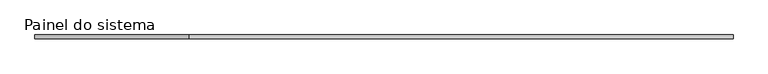
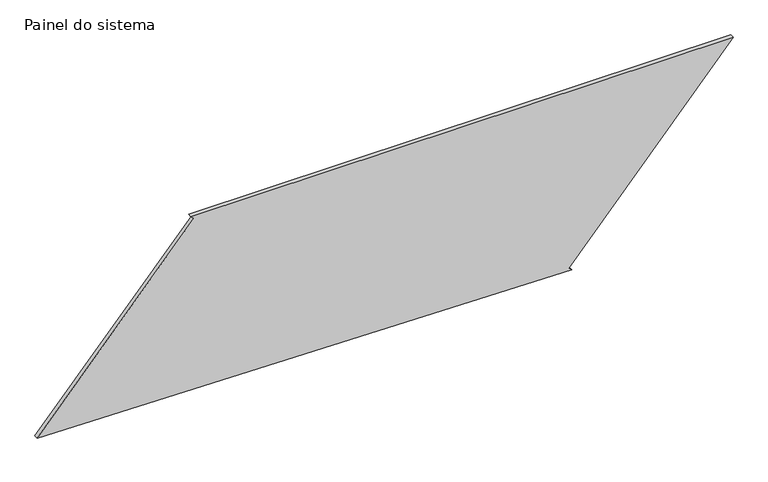
"""IFC4 building model written with IfcOpenShell, lengths in millimetres: plate geometry, Painel do sistema : Envidraçado."""

from ifc_helpers import new_model, si_unit, frame, origin, place, context, project, spatial, polyline, outline, extrude, source, transform, mapped, element, save


def painel_do_sistema_3713dc80(model_context):
    return source(origin(), model_context, "Body", "SweptSolid", [
        extrude(outline(polyline([(0.0, 1167.9821975), (16.5356636, 1149.2319488), (1185.4896941, 2180.1212412), (1185.4896941, -1216.67228), (1168.9540304, -1197.9220313), (55.2110382, -2180.1212412), (0.0, 1167.9821975)])), frame((0.0, 24.5, 0.0), z_axis=(0.0, 1.0, 0.0), x_axis=(0.0, 0.0, 1.0)), (0.0, 0.0, 1.0), 25.0),
    ])


if __name__ == "__main__":
    model = new_model("IFC4")
    model_context = context("Model", 3, world=origin())
    ifc_project = project(units=[si_unit("LENGTHUNIT", "METRE", prefix="MILLI")], contexts=[model_context])
    site = spatial("IfcSite", under=ifc_project)
    building = spatial("IfcBuilding", under=site)
    placement = place(None, origin())
    painel_do_sistema_shape = painel_do_sistema_3713dc80(model_context)
    element("IfcPlate", 1, ObjectType="Painel do sistema : Envidraçado", at=placement, inside=building, context=model_context, shape_type="MappedRepresentation", body=[
        mapped(painel_do_sistema_shape, transform((0.0, 0.0, 0.0), x_axis=(1.0, 0.0, 0.0), y_axis=(0.0, 1.0, 0.0), z_axis=(0.0, 0.0, 1.0))),
    ])
    save(model, "model.ifc")

# Revit data of these elements
# Type "Painel do sistema : Envidraçado"
#   Construction Type Id = "GSP4R"
#   Analytic Construction = "Vidraça única Pilkington 1/8 pol"
#   Visual Light Transmittance = 0.9
#   Solar Heat Gain Coefficient = 0.86
#   Heat Transfer Coefficient (U) = 6.7069 W/(m²·K)
# Element 1 (IfcPlate, "Painel do sistema : Envidraçado")
#   Materials on its faces: "Vidro"
# Materials
#   "Vidro": class "Vidro", colour RGB 0 128 192, transparency 0.9, Description = "Vidro de sílica", Cost = 0
